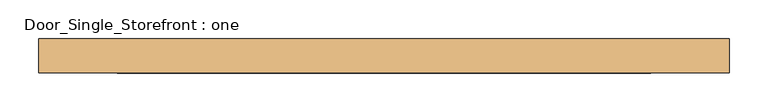
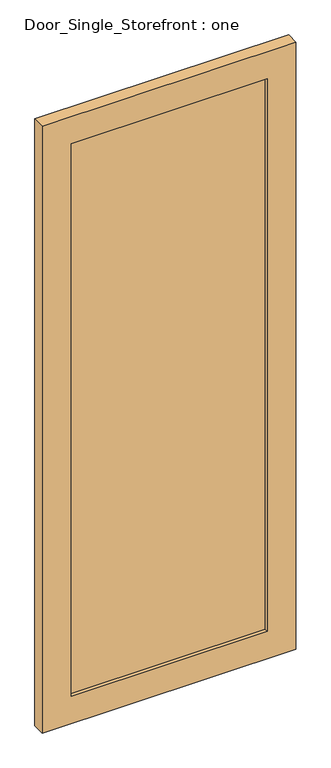
"""IFC4 building model written with IfcOpenShell, lengths in millimetres: door geometry, Door_Single_Storefront : one."""

import ifcopenshell
import ifcopenshell.guid

model = None  # the IFC model being written
_history = None  # IfcOwnerHistory: only IFC2X3 demands one
_inside = {}  # id of a spatial element -> (the spatial element, [elements in it])
_under = {}  # id of a project, library or spatial element -> (it, [spatial elements below it])
_declared = {}  # id of a project -> (the project, [libraries it declares])
_typed = {}  # id of a type object -> (the type object, [elements of that type])
_made_of = {}  # id of a material, layer set ... -> (it, [elements and type objects made of it])


def new_model(schema):
    """Start an empty IFC model of exactly this schema.

    Asked for "IFC4X3", IfcOpenShell would pick the latest addendum, in which some entities
    have other attributes; the version numbers below select the first issue.
    IFC2X3 requires an IfcOwnerHistory on every rooted entity: one is made here for all.
    """
    global model, _history
    if schema == "IFC4X3":
        model = ifcopenshell.file(schema_version=(4, 3, 0, 0))
    else:
        model = ifcopenshell.file(schema=schema)
    _inside.clear()
    _under.clear()
    _declared.clear()
    _typed.clear()
    _made_of.clear()
    _history = None
    if model.schema == "IFC2X3":
        org = make("IfcOrganization", Name="unknown")
        user = make(
            "IfcPersonAndOrganization",
            ThePerson=make("IfcPerson", FamilyName="unknown"),
            TheOrganization=org,
        )
        app = make(
            "IfcApplication",
            ApplicationDeveloper=org,
            Version="unknown",
            ApplicationFullName="unknown",
            ApplicationIdentifier="unknown",
        )
        _history = make(
            "IfcOwnerHistory",
            OwningUser=user,
            OwningApplication=app,
            ChangeAction="ADDED",
            CreationDate=0,
        )
    return model


def make(cls, **values):
    """One entity of the class cls with the attributes given. An attribute that is None is left unset."""
    return model.create_entity(
        cls, **{name: value for name, value in values.items() if value is not None}
    )


def rooted(cls, **values):
    """An entity with a GlobalId (a new one), such as an element, a storey or a relation."""
    return make(cls, GlobalId=ifcopenshell.guid.new(), OwnerHistory=_history, **values)


def si_unit(unit_type, name, prefix=None):
    """IfcSIUnit, for example si_unit("LENGTHUNIT", "METRE", prefix="MILLI")."""
    return make("IfcSIUnit", UnitType=unit_type, Prefix=prefix, Name=name)


def assignment(units):
    """IfcUnitAssignment: the units of a project."""
    return None if units is None else make("IfcUnitAssignment", Units=units)


def point(xyz):
    """IfcCartesianPoint."""
    return None if xyz is None else make("IfcCartesianPoint", Coordinates=xyz)


def direction(xyz):
    """IfcDirection."""
    return None if xyz is None else make("IfcDirection", DirectionRatios=xyz)


def frame(location, z_axis=None, x_axis=None):
    """IfcAxis2Placement3D, a coordinate frame: its origin and axes. An axis left out is left unset."""
    return make(
        "IfcAxis2Placement3D",
        Location=point(location),
        Axis=direction(z_axis),
        RefDirection=direction(x_axis),
    )


def origin():
    """The frame at (0, 0, 0) with its axes left unset."""
    return frame((0.0, 0.0, 0.0))


def place(relative_to, where):
    """IfcLocalPlacement: puts the frame where relative to a parent placement (None: the world)."""
    return make(
        "IfcLocalPlacement", PlacementRelTo=relative_to, RelativePlacement=where
    )


def context(
    kind, dimensions, precision=None, world=None, true_north=None, identifier=None
):
    """IfcGeometricRepresentationContext, for example the 3D "Model" context."""
    return make(
        "IfcGeometricRepresentationContext",
        ContextIdentifier=identifier,
        ContextType=kind,
        CoordinateSpaceDimension=dimensions,
        Precision=precision,
        WorldCoordinateSystem=world,
        TrueNorth=true_north,
    )


def project(units=None, contexts=None):
    """IfcProject with its units and contexts."""
    return rooted(
        "IfcProject",
        Name="project",
        RepresentationContexts=contexts,
        UnitsInContext=assignment(units),
    )


def spatial(cls, under=None, at=None, **own):
    """A site, building, storey or space (cls), placed at a placement, below another one or the project."""
    s = rooted(cls, ObjectPlacement=at, **own)
    if under is not None:
        _under.setdefault(under.id(), (under, []))[1].append(s)
    return s


def polyline(points):
    """IfcPolyline through the points."""
    return make("IfcPolyline", Points=[point(p) for p in points])


def outline(outer, holes=None, kind="AREA"):
    """IfcArbitraryClosedProfileDef: a profile drawn as a closed curve; with holes, ...WithVoids."""
    if holes is None:
        return make("IfcArbitraryClosedProfileDef", ProfileType=kind, OuterCurve=outer)
    return make(
        "IfcArbitraryProfileDefWithVoids",
        ProfileType=kind,
        OuterCurve=outer,
        InnerCurves=holes,
    )


def extrude(swept, where, along, depth):
    """IfcExtrudedAreaSolid: the profile swept, set in the frame where, extruded along a direction by depth."""
    return make(
        "IfcExtrudedAreaSolid",
        SweptArea=swept,
        Position=where,
        ExtrudedDirection=direction(along),
        Depth=depth,
    )


def shape(context_of_items, identifier, shape_type, items):
    """IfcShapeRepresentation: the items that make up one representation, for example the "Body"."""
    return make(
        "IfcShapeRepresentation",
        ContextOfItems=context_of_items,
        RepresentationIdentifier=identifier,
        RepresentationType=shape_type,
        Items=items,
    )


def source(mapping_origin, context_of_items, identifier, shape_type, items):
    """IfcRepresentationMap: a shape defined once, which mapped items show again and again."""
    return make(
        "IfcRepresentationMap",
        MappingOrigin=mapping_origin,
        MappedRepresentation=shape(context_of_items, identifier, shape_type, items),
    )


def transform(
    local_origin,
    x_axis=None,
    y_axis=None,
    z_axis=None,
    scale=None,
    scale2=None,
    scale3=None,
    uniform=True,
):
    """IfcCartesianTransformationOperator3D, or its non-uniform kind. x_axis, y_axis, z_axis: its Axis1, 2, 3."""
    if uniform:
        return make(
            "IfcCartesianTransformationOperator3D",
            Axis1=direction(x_axis),
            Axis2=direction(y_axis),
            LocalOrigin=point(local_origin),
            Scale=scale,
            Axis3=direction(z_axis),
        )
    return make(
        "IfcCartesianTransformationOperator3DnonUniform",
        Axis1=direction(x_axis),
        Axis2=direction(y_axis),
        LocalOrigin=point(local_origin),
        Scale=scale,
        Axis3=direction(z_axis),
        Scale2=scale2,
        Scale3=scale3,
    )


def mapped(mapping_source, mapping_target):
    """IfcMappedItem: shows the shape of a source again, moved by a transform."""
    return make(
        "IfcMappedItem", MappingSource=mapping_source, MappingTarget=mapping_target
    )


def made_of(thing, what):
    """Note that an element or type object is made of a material, layer set ...; save() writes the relation."""
    if what is not None:
        _made_of.setdefault(what.id(), (what, []))[1].append(thing)
    return thing


def element(
    cls,
    number,
    at=None,
    inside=None,
    cuts=None,
    type_object=None,
    material=None,
    context=None,
    identifier="Body",
    shape_type=None,
    held_by="IfcProductDefinitionShape",
    body=None,
    shapes=None,
    **own,
):
    """One element of the class cls, such as IfcWall. Its Tag is "e" and its number.

    at: its placement. inside: the storey or other place that contains it. cuts: it is an
    opening in that element (IfcRelVoidsElement). A single representation is given by context,
    identifier, shape_type and body (its items); several are given by shapes. held_by: the class
    of the entity that holds the representations. save() writes the other relations.
    """
    e = rooted(cls, Tag="e%d" % number, ObjectPlacement=at, **own)
    if body is not None:
        shapes = [shape(context, identifier, shape_type, body)]
    if shapes is not None:
        e.Representation = make(held_by, Representations=shapes)
    if inside is not None:
        _inside.setdefault(inside.id(), (inside, []))[1].append(e)
    if cuts is not None:
        rooted(
            "IfcRelVoidsElement", RelatingBuildingElement=cuts, RelatedOpeningElement=e
        )
    if type_object is not None:
        _typed.setdefault(type_object.id(), (type_object, []))[1].append(e)
    return made_of(e, material)


def aggregate(whole, parts):
    """IfcRelAggregates: a whole, such as a stair, and the parts it consists of."""
    return rooted("IfcRelAggregates", RelatingObject=whole, RelatedObjects=parts)


def save(model, path):
    """Write the relations noted so far, then the file.

    IfcRelAggregates (storeys below a building ...), IfcRelContainedInSpatialStructure (elements
    in a storey), IfcRelDefinesByType, IfcRelAssociatesMaterial and IfcRelDeclares: one each for
    every whole, place, type object, material and project.
    """
    for whole, parts in _under.values():
        aggregate(whole, parts)
    for where, things in _inside.values():
        rooted(
            "IfcRelContainedInSpatialStructure",
            RelatedElements=things,
            RelatingStructure=where,
        )
    for kind, things in _typed.values():
        rooted("IfcRelDefinesByType", RelatedObjects=things, RelatingType=kind)
    for what, things in _made_of.values():
        rooted("IfcRelAssociatesMaterial", RelatedObjects=things, RelatingMaterial=what)
    for by, libraries in _declared.values():
        rooted("IfcRelDeclares", RelatingContext=by, RelatedDefinitions=libraries)
    model.write(path)


def door_single_storefront_one_3d44b09d(model_context):
    return source(origin(), model_context, "Body", "SweptSolid", [
        extrude(outline(polyline([(345.28125, 6.35), (345.28125, -12.7), (-345.28125, -12.7), (-345.28125, 6.35), (345.28125, 6.35)])), frame((0.0, 0.0, 101.6), z_axis=(0.0, 0.0, 1.0), x_axis=(1.0, 0.0, 0.0)), (0.0, 0.0, 1.0), 2057.4),
        extrude(outline(polyline([(2260.6, -446.88125), (0.0, -446.88125), (0.0, 446.88125), (2260.6, 446.88125), (2260.6, -446.88125)]), holes=[polyline([(101.6, 345.28125), (101.6, -345.28125), (2159.0, -345.28125), (2159.0, 345.28125), (101.6, 345.28125)])]), frame((0.0, -25.4, 0.0), z_axis=(0.0, 1.0, 0.0), x_axis=(0.0, 0.0, 1.0)), (0.0, 0.0, 1.0), 44.45),
    ])


if __name__ == "__main__":
    model = new_model("IFC4")
    model_context = context("Model", 3, world=origin())
    ifc_project = project(units=[si_unit("LENGTHUNIT", "METRE", prefix="MILLI")], contexts=[model_context])
    site = spatial("IfcSite", under=ifc_project)
    building = spatial("IfcBuilding", under=site)
    placement = place(None, origin())
    door_single_storefront_one_shape = door_single_storefront_one_3d44b09d(model_context)
    element("IfcDoor", 1, ObjectType="Door_Single_Storefront : one", at=placement, inside=building, context=model_context, shape_type="MappedRepresentation", body=[
        mapped(door_single_storefront_one_shape, transform((0.0, 0.0, 0.0), x_axis=(1.0, 0.0, 0.0), y_axis=(0.0, 1.0, 0.0), z_axis=(0.0, 0.0, 1.0))),
    ])
    save(model, "model.ifc")

# Revit data of these elements
# Type "Door_Single_Storefront : one"
#   Type Mark = "27"
#   Analytic Construction = "<None>"
#   Stile_Width = 0' - 4"
#   Door_Thickness = 0' - 1 3/4"
#   Door_Offset = 0' - 1"
#   Glass_Material = Glass
#   Frame_Material = Aluminum
#   Function = (empty or 0)
# Element 1 (IfcDoor, "Door_Single_Storefront : one")
#   Materials on its faces: "Aluminum", "Glass"
# Materials
#   "Glass": class "Glass", colour RGB 142 168 196, transparency 0.75, Description = "Soda Lime Glass", Cost = 0
#   "Aluminum": class "Metal", colour RGB 226 226 226, transparency 0, Description = "Aluminum 6061", Cost = 0
